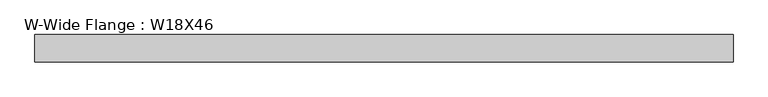
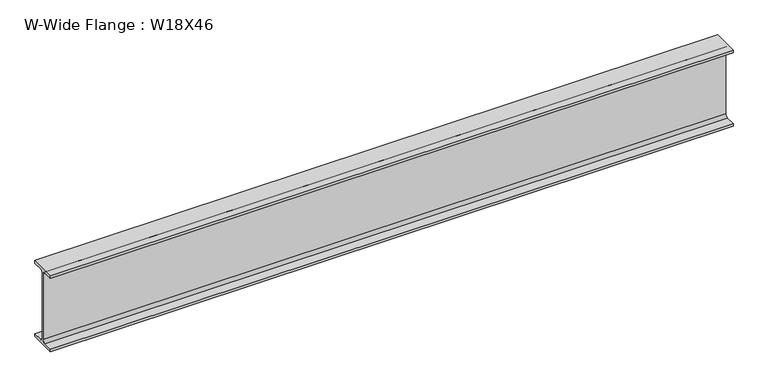
"""IFC4 building model written with IfcOpenShell, lengths in millimetres: beam geometry, W-Wide Flange : W18X46."""

from ifc_helpers import new_model, si_unit, point, frame, frame_2d, origin, place, context, project, spatial, polyline, circle_curve, trimmed, segment, composite_curve, outline, extrude, source, transform, mapped, element, save


def w_wide_flange_w18x46_72a3854d(model_context):
    return source(origin(), model_context, "Body", "SweptSolid", [
        extrude(outline(composite_curve([segment(polyline([(76.962, -214.503), (76.962, -229.87), (-76.962, -229.87), (-76.962, -214.503), (-20.955, -214.503)]), True, "CONTINUOUS"), segment(trimmed(circle_curve(frame_2d((-20.955, -198.12)), 16.383), [point((-20.955, -214.503))], [point((-4.572, -198.12))], True, "CARTESIAN"), True, "CONTINUOUS"), segment(polyline([(-4.572, -198.12), (-4.572, 198.12)]), True, "CONTINUOUS"), segment(trimmed(circle_curve(frame_2d((-20.955, 198.12)), 16.383), [point((-4.572, 198.12))], [point((-20.955, 214.503))], True, "CARTESIAN"), True, "CONTINUOUS"), segment(polyline([(-20.955, 214.503), (-76.962, 214.503), (-76.962, 229.87), (76.962, 229.87), (76.962, 214.503), (20.955, 214.503)]), True, "CONTINUOUS"), segment(trimmed(circle_curve(frame_2d((20.955, 198.12)), 16.383), [point((20.955, 214.503))], [point((4.572, 198.12))], True, "CARTESIAN"), True, "CONTINUOUS"), segment(polyline([(4.572, 198.12), (4.572, -198.12)]), True, "CONTINUOUS"), segment(trimmed(circle_curve(frame_2d((20.955, -198.12)), 16.383), [point((4.572, -198.12))], [point((20.955, -214.503))], True, "CARTESIAN"), True, "CONTINUOUS"), segment(polyline([(20.955, -214.503), (76.962, -214.503)]), True, "CONTINUOUS")], self_intersect=False)), frame((-1955.8, 0.0, 0.0), z_axis=(1.0, 0.0, 0.0), x_axis=(0.0, 1.0, 0.0)), (0.0, 0.0, 1.0), 3911.6),
    ])


if __name__ == "__main__":
    model = new_model("IFC4")
    model_context = context("Model", 3, world=origin())
    ifc_project = project(units=[si_unit("LENGTHUNIT", "METRE", prefix="MILLI")], contexts=[model_context])
    site = spatial("IfcSite", under=ifc_project)
    building = spatial("IfcBuilding", under=site)
    placement = place(None, origin())
    w_wide_flange_w18x46_shape = w_wide_flange_w18x46_72a3854d(model_context)
    element("IfcBeam", 1, ObjectType="W-Wide Flange : W18X46", at=placement, inside=building, context=model_context, shape_type="MappedRepresentation", body=[
        mapped(w_wide_flange_w18x46_shape, transform((0.0, 0.0, 0.0), x_axis=(1.0, 0.0, 0.0), y_axis=(0.0, 1.0, 0.0), z_axis=(0.0, 0.0, 1.0))),
    ])
    save(model, "model.ifc")

# Revit data of these elements
# Type "W-Wide Flange : W18X46"
#   Assembly Code = "B10"
#   W = 46
#   Length [instance default] = 5' - 0"
#   bf = 0' - 6.06"
#   d = 1' - 6.1"
#   k = 0' - 1 1/4"
#   k2 = 0' - 0.645"
#   tf = 0' - 0.605"
#   tw = 0' - 0.36"
#   A = 0.09375 SF
#   Structural Material [instance default] = Steel ASTM A992
# Element 1 (IfcBeam, "W-Wide Flange : W18X46")
#   Materials on its faces: "Steel ASTM A992"
# Materials
#   "Steel ASTM A992": class "Metal", colour RGB 199 199 199, transparency 0, Description = "Structural steel 50ksi", Cost = 0
